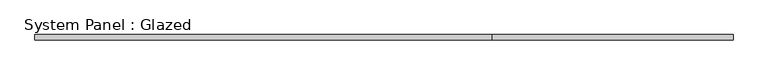
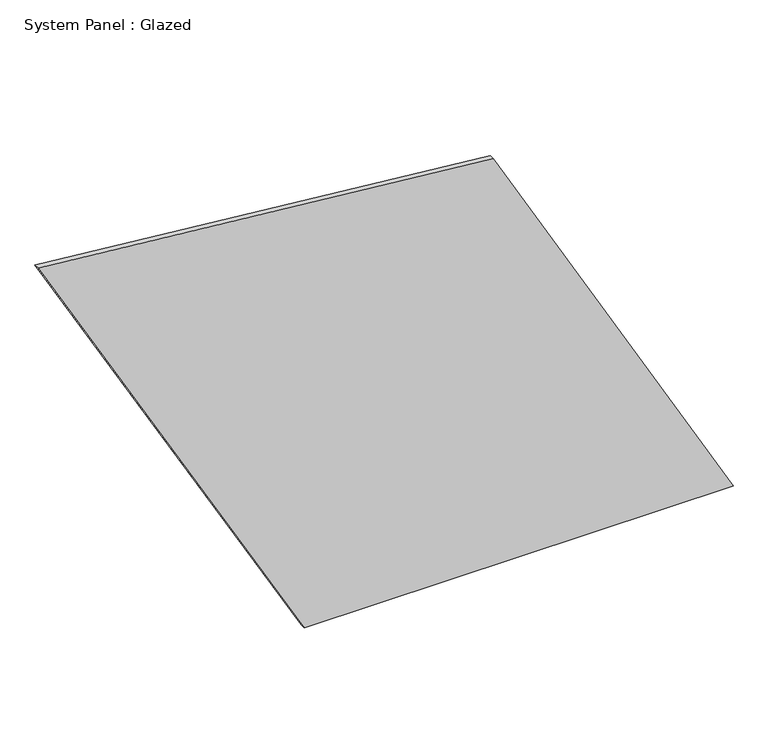
"""IFC4 building model written with IfcOpenShell, lengths in millimetres: plate geometry, System Panel : Glazed."""

from ifc_helpers import new_model, si_unit, frame, origin, place, context, project, spatial, polyline, outline, extrude, source, transform, mapped, element, save


def system_panel_glazed_27796991(model_context):
    return source(origin(), model_context, "Body", "SweptSolid", [
        extrude(outline(polyline([(0.0, -375.3783473), (0.0, 1602.1783299), (1983.3983462, 496.8878849), (2185.1781976, -1602.1783299), (0.0, -375.3783473)])), frame((0.0, -49.5, 0.0), z_axis=(0.0, 1.0, 0.0), x_axis=(0.0, 0.0, 1.0)), (0.0, 0.0, 1.0), 25.0),
    ])


if __name__ == "__main__":
    model = new_model("IFC4")
    model_context = context("Model", 3, world=origin())
    ifc_project = project(units=[si_unit("LENGTHUNIT", "METRE", prefix="MILLI")], contexts=[model_context])
    site = spatial("IfcSite", under=ifc_project)
    building = spatial("IfcBuilding", under=site)
    placement = place(None, origin())
    system_panel_glazed_shape = system_panel_glazed_27796991(model_context)
    element("IfcPlate", 1, ObjectType="System Panel : Glazed", at=placement, inside=building, context=model_context, shape_type="MappedRepresentation", body=[
        mapped(system_panel_glazed_shape, transform((0.0, 0.0, 0.0), x_axis=(1.0, 0.0, 0.0), y_axis=(0.0, 1.0, 0.0), z_axis=(0.0, 0.0, 1.0))),
    ])
    save(model, "model.ifc")

# Revit data of these elements
# Element 1 (IfcPlate, "System Panel : Glazed")
#   Materials on its faces: "Glass, Clear Glazing"
# Materials
#   "Glass, Clear Glazing": class "Glass", colour RGB 247 249 248, transparency 0.85, Description = "Clear glazing", Cost = 0
